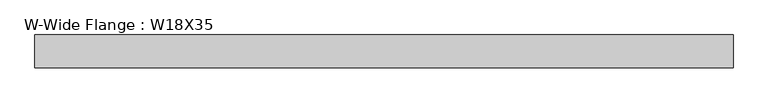
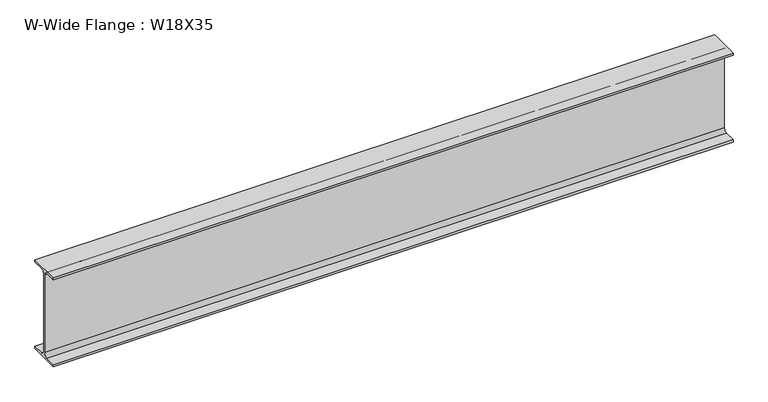
"""IFC4 building model written with IfcOpenShell, lengths in millimetres: beam geometry, W-Wide Flange : W18X35."""

from ifc_helpers import new_model, si_unit, point, frame, frame_2d, origin, place, context, project, spatial, polyline, circle_curve, trimmed, segment, composite_curve, outline, extrude, source, transform, mapped, element, save


def w_wide_flange_w18x35_57d56bca(model_context):
    return source(origin(), model_context, "Body", "SweptSolid", [
        extrude(outline(composite_curve([segment(polyline([(76.2, -213.995), (76.2, -224.79), (-76.2, -224.79), (-76.2, -213.995), (-21.59, -213.995)]), True, "CONTINUOUS"), segment(trimmed(circle_curve(frame_2d((-21.59, -196.215)), 17.78), [point((-21.59, -213.995))], [point((-3.81, -196.215))], True, "CARTESIAN"), True, "CONTINUOUS"), segment(polyline([(-3.81, -196.215), (-3.81, 196.215)]), True, "CONTINUOUS"), segment(trimmed(circle_curve(frame_2d((-21.59, 196.215)), 17.78), [point((-3.81, 196.215))], [point((-21.59, 213.995))], True, "CARTESIAN"), True, "CONTINUOUS"), segment(polyline([(-21.59, 213.995), (-76.2, 213.995), (-76.2, 224.79), (76.2, 224.79), (76.2, 213.995), (21.59, 213.995)]), True, "CONTINUOUS"), segment(trimmed(circle_curve(frame_2d((21.59, 196.215)), 17.78), [point((21.59, 213.995))], [point((3.81, 196.215))], True, "CARTESIAN"), True, "CONTINUOUS"), segment(polyline([(3.81, 196.215), (3.81, -196.215)]), True, "CONTINUOUS"), segment(trimmed(circle_curve(frame_2d((21.59, -196.215)), 17.78), [point((3.81, -196.215))], [point((21.59, -213.995))], True, "CARTESIAN"), True, "CONTINUOUS"), segment(polyline([(21.59, -213.995), (76.2, -213.995)]), True, "CONTINUOUS")], self_intersect=False)), frame((-1625.6, 0.0, 0.0), z_axis=(1.0, 0.0, 0.0), x_axis=(0.0, 1.0, 0.0)), (0.0, 0.0, 1.0), 3251.2),
    ])


if __name__ == "__main__":
    model = new_model("IFC4")
    model_context = context("Model", 3, world=origin())
    ifc_project = project(units=[si_unit("LENGTHUNIT", "METRE", prefix="MILLI")], contexts=[model_context])
    site = spatial("IfcSite", under=ifc_project)
    building = spatial("IfcBuilding", under=site)
    placement = place(None, origin())
    w_wide_flange_w18x35_shape = w_wide_flange_w18x35_57d56bca(model_context)
    element("IfcBeam", 1, ObjectType="W-Wide Flange : W18X35", at=placement, inside=building, context=model_context, shape_type="MappedRepresentation", body=[
        mapped(w_wide_flange_w18x35_shape, transform((0.0, 0.0, 0.0), x_axis=(1.0, 0.0, 0.0), y_axis=(0.0, 1.0, 0.0), z_axis=(0.0, 0.0, 1.0))),
    ])
    save(model, "model.ifc")

# Revit data of these elements
# Type "W-Wide Flange : W18X35"
#   Assembly Code = "B10"
#   W = 35
#   Length [instance default] = 5' - 0"
#   bf = 0' - 6"
#   d = 1' - 5.7"
#   k = 0' - 1 1/8"
#   k2 = 0' - 0.7"
#   tf = 0' - 0.425"
#   tw = 0' - 0.3"
#   A = 0.0715278 SF
#   Structural Material [instance default] = Steel ASTM A992
# Element 1 (IfcBeam, "W-Wide Flange : W18X35")
#   Materials on its faces: "Steel ASTM A992"
# Materials
#   "Steel ASTM A992": class "Metal", colour RGB 199 199 199, transparency 0, Description = "Structural steel 50ksi", Cost = 0
